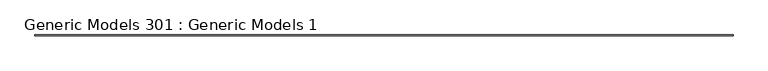
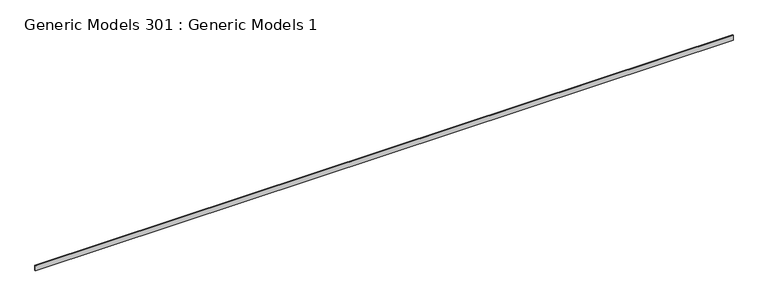
"""IFC4 building model written with IfcOpenShell, lengths in millimetres: proxy geometry, Generic Models 301 : Generic Models 1."""

from ifc_helpers import new_model, si_unit, frame, origin, place, context, project, spatial, polyline, outline, extrude, source, transform, mapped, element, save


def generic_models_301_generic_models_1_a2a94731(model_context):
    return source(origin(), model_context, "Body", "SweptSolid", [
        extrude(outline(polyline([(11204.7748879, 126896.2722833), (11204.7748879, 127034.7816583), (11205.9655129, 127035.9722833), (11223.8248879, 127035.9722833), (11223.8248879, 126896.2722833), (11204.7748879, 126896.2722833)])), frame((-10437.7171316, 0.0, 0.0), z_axis=(1.0, 0.0, 0.0), x_axis=(0.0, 1.0, 0.0)), (0.0, 0.0, 1.0), 19050.0),
    ])


if __name__ == "__main__":
    model = new_model("IFC4")
    model_context = context("Model", 3, world=origin())
    ifc_project = project(units=[si_unit("LENGTHUNIT", "METRE", prefix="MILLI")], contexts=[model_context])
    site = spatial("IfcSite", under=ifc_project)
    building = spatial("IfcBuilding", under=site)
    placement = place(None, origin())
    generic_models_301_generic_models_1_shape = generic_models_301_generic_models_1_a2a94731(model_context)
    element("IfcBuildingElementProxy", 1, Name="Generic Models 301 : Generic Models 1", ObjectType="Generic Models 301 : Generic Models 1", at=placement, inside=building, context=model_context, shape_type="MappedRepresentation", body=[
        mapped(generic_models_301_generic_models_1_shape, transform((0.0, 0.0, 0.0), x_axis=(1.0, 0.0, 0.0), y_axis=(0.0, 1.0, 0.0), z_axis=(0.0, 0.0, 1.0))),
    ])
    save(model, "model.ifc")

# Revit data of these elements
# Element 1 (IfcBuildingElementProxy, "Generic Models 301 : Generic Models 1")
#   Materials on its faces: "_BASE TRIM AS SCHEDULED"
# Materials
#   "_BASE TRIM AS SCHEDULED": class "Generic", colour RGB 177 130 114, transparency 0, Cost = 0
